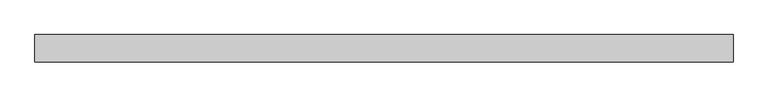
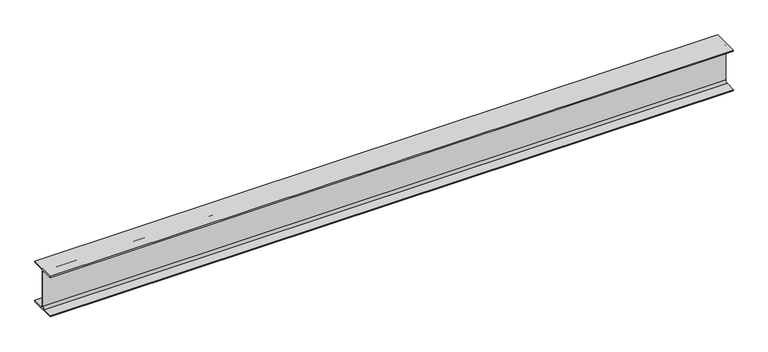
"""IFC4 building model written with IfcOpenShell, lengths in millimetres: beam geometry, 0912_Steel Framing_H-KSD3502 : H_SB_ASB_H-482x300x11x15."""

from ifc_helpers import new_model, si_unit, point, frame, frame_2d, origin, place, context, project, spatial, polyline, circle_curve, trimmed, segment, composite_curve, outline, extrude, source, transform, mapped, element, save


def beam_c5fb2c0c(model_context):
    return source(origin(), model_context, "Body", "SweptSolid", [
        extrude(outline(composite_curve([segment(polyline([(150.0, -226.0), (150.0, -241.0), (-150.0, -241.0), (-150.0, -226.0), (-31.5, -226.0)]), True, "CONTINUOUS"), segment(trimmed(circle_curve(frame_2d((-31.5, -200.0)), 26.0), [point((-31.5, -226.0))], [point((-5.5, -200.0))], True, "CARTESIAN"), True, "CONTINUOUS"), segment(polyline([(-5.5, -200.0), (-5.5, 200.0)]), True, "CONTINUOUS"), segment(trimmed(circle_curve(frame_2d((-31.5, 200.0)), 26.0), [point((-5.5, 200.0))], [point((-31.5, 226.0))], True, "CARTESIAN"), True, "CONTINUOUS"), segment(polyline([(-31.5, 226.0), (-150.0, 226.0), (-150.0, 241.0), (150.0, 241.0), (150.0, 226.0), (31.5, 226.0)]), True, "CONTINUOUS"), segment(trimmed(circle_curve(frame_2d((31.5, 200.0)), 26.0), [point((31.5, 226.0))], [point((5.5, 200.0))], True, "CARTESIAN"), True, "CONTINUOUS"), segment(polyline([(5.5, 200.0), (5.5, -200.0)]), True, "CONTINUOUS"), segment(trimmed(circle_curve(frame_2d((31.5, -200.0)), 26.0), [point((5.5, -200.0))], [point((31.5, -226.0))], True, "CARTESIAN"), True, "CONTINUOUS"), segment(polyline([(31.5, -226.0), (150.0, -226.0)]), True, "CONTINUOUS")], self_intersect=False)), frame((-3837.3, 0.0, 0.0), z_axis=(1.0, 0.0, 0.0), x_axis=(0.0, 1.0, 0.0)), (0.0, 0.0, 1.0), 7674.6),
    ])


if __name__ == "__main__":
    model = new_model("IFC4")
    model_context = context("Model", 3, world=origin())
    ifc_project = project(units=[si_unit("LENGTHUNIT", "METRE", prefix="MILLI")], contexts=[model_context])
    site = spatial("IfcSite", under=ifc_project)
    building = spatial("IfcBuilding", under=site)
    placement = place(None, origin())
    beam_shape = beam_c5fb2c0c(model_context)
    element("IfcBeam", 1, ObjectType="0912_Steel Framing_H-KSD3502 : H_SB_ASB_H-482x300x11x15", at=placement, inside=building, context=model_context, shape_type="MappedRepresentation", body=[
        mapped(beam_shape, transform((0.0, 0.0, 0.0), x_axis=(1.0, 0.0, 0.0), y_axis=(0.0, 1.0, 0.0), z_axis=(0.0, 0.0, 1.0))),
    ])
    save(model, "model.ifc")

# Revit data of these elements
# Type "0912_Steel Framing_H-KSD3502 : H_SB_ASB_H-482x300x11x15"
#   H_WM Code_1 = "S01AA001-00001 | Main Steel Structure Fabrication Work | Shelter/Building | Heavy Steel - Standard (Weight≥90KG/M) | Material: (   )"
#   H_WM Code_2 = "S03AA027-00001 | Main Steel Structure Erection Work | Shelter/Building | Heavy Steel (Weight≥90KG/M) | Material: (   )"
#   H_WM Code_3 = "S01AA010-00001 | Main Steel Structure Fabrication Work | Shelter/Building | Steel Painting/Coating | for Non-Fireproofed Steel Surface, Surface Preparation, Primer, Second & Final Coat | Material: (   )"
#   H_Q'ty Cal Type Tag = "SB-Q2"
#   Width = 30.0 cm
#   Web Thickness = 1.1 cm
#   Web Fillet = 2.6 cm
#   Warping Constant = 3680000.0 cm⁶
#   W = 0
#   Torsional Moment of Inertia = 88.2192 cm⁴
#   Section Area = 145.5 cm²
#   Plastic Modulus weak axis = 695.0 cm³
#   Plastic Modulus strong axis = 2790.0 cm³
#   Perimeter = 2.10 m²/m
#   Nominal Weight = 114.00 kgf/m
#   Moment of Inertia weak axis = 6760.00 cm⁴
#   Moment of Inertia strong axis = 60400.00 cm⁴
#   Height = 48.2 cm
#   Flange Thickness = 1.5 cm
#   Elastic Modulus weak axis = 451.0 cm³
#   Elastic Modulus strong axis = 2500.0 cm³
#   Centroid Vertical = 24.1 cm
#   Centroid Horizontal = 15.0 cm
#   Ix = 604000000
#   Length [instance default] = 1.5240 m
#   Zx = 2790000
#   b = 0.3000 m
#   h = 0.4820 m
#   r = 0.0260 m
#   s = 0.0110 m
#   t = 0.0150 m
#   A = 0.01455 m²
#   Structural Material [instance default] = Steel, 45-345
#   Assembly Code = ""
# Element 1 (IfcBeam, "0912_Steel Framing_H-KSD3502 : H_SB_ASB_H-482x300x11x15")
#   Structural Material = none
# Materials
#   "Steel, 45-345": class "Metal", colour RGB 189 187 185, transparency 0, Description = "Steel 345 MPa", Cost = 0
